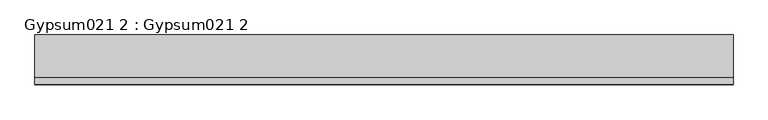
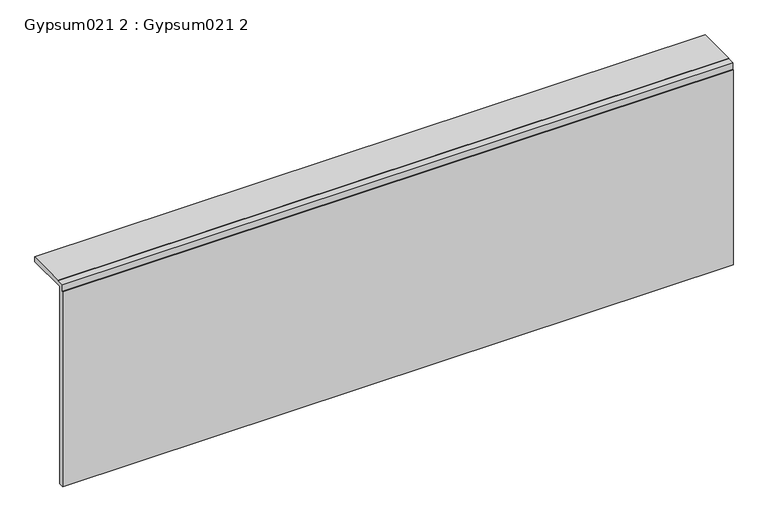
"""IFC4 building model written with IfcOpenShell, lengths in millimetres: proxy geometry, Gypsum021 2 : Gypsum021 2."""

from ifc_helpers import new_model, si_unit, frame, origin, place, context, project, spatial, polyline, outline, extrude, source, transform, mapped, element, save


def gypsum021_2_gypsum021_2_57715f0e(model_context):
    return source(origin(), model_context, "Body", "SweptSolid", [
        extrude(outline(polyline([(10284.5464235, 40795.72275), (10405.3424948, 40795.72275), (10405.3424948, 40779.84775), (10277.9882396, 40779.84775), (10277.9882396, 40157.1516563), (10262.1132396, 40157.1516563), (10262.1132396, 40773.2895661), (10263.3932396, 40773.2895661), (10263.3932396, 40794.44275), (10284.5464235, 40794.44275), (10284.5464235, 40795.72275)])), frame((3694.2883192, 0.0, 0.0), z_axis=(1.0, 0.0, 0.0), x_axis=(0.0, 1.0, 0.0)), (0.0, 0.0, 1.0), 2000.25),
    ])


if __name__ == "__main__":
    model = new_model("IFC4")
    model_context = context("Model", 3, world=origin())
    ifc_project = project(units=[si_unit("LENGTHUNIT", "METRE", prefix="MILLI")], contexts=[model_context])
    site = spatial("IfcSite", under=ifc_project)
    building = spatial("IfcBuilding", under=site)
    placement = place(None, origin())
    gypsum021_2_gypsum021_2_shape = gypsum021_2_gypsum021_2_57715f0e(model_context)
    element("IfcBuildingElementProxy", 1, Name="Gypsum021 2 : Gypsum021 2", ObjectType="Gypsum021 2 : Gypsum021 2", at=placement, inside=building, context=model_context, shape_type="MappedRepresentation", body=[
        mapped(gypsum021_2_gypsum021_2_shape, transform((0.0, 0.0, 0.0), x_axis=(1.0, 0.0, 0.0), y_axis=(0.0, 1.0, 0.0), z_axis=(0.0, 0.0, 1.0))),
    ])
    save(model, "model.ifc")

# Revit data of these elements
# Type "Gypsum021 2 : Gypsum021 2"
#   NameOverride = "Gypsum021"
# Element 1 (IfcBuildingElementProxy, "Gypsum021 2 : Gypsum021 2")
#   Materials on its faces: "5/8\"  GYPSUM BOARD"
# Materials
#   "5/8\"  GYPSUM BOARD": class "Unassigned", colour RGB 255 255 255, transparency 0, Cost = 0
